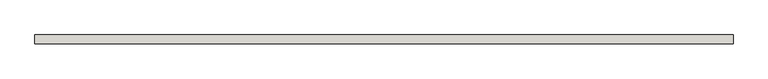
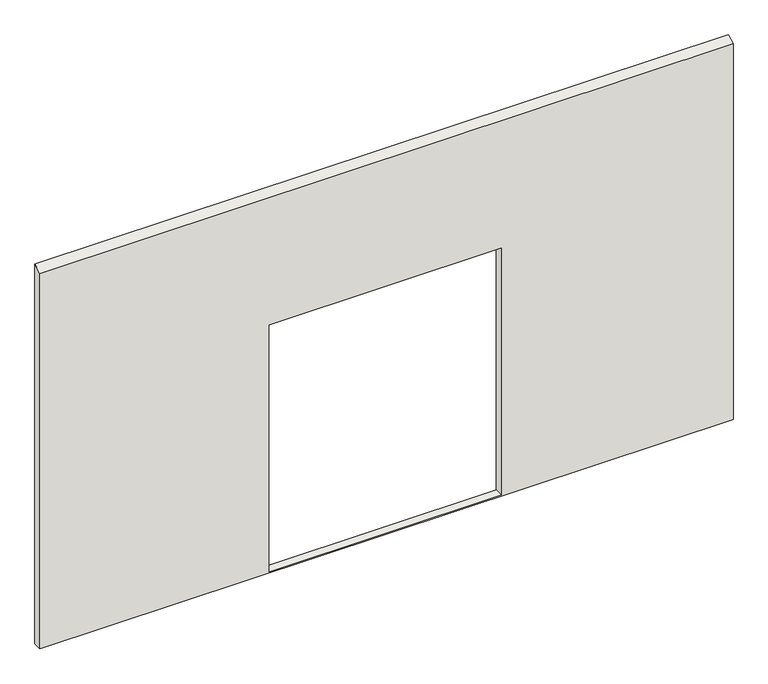
"""IFC4 building model written with IfcOpenShell, lengths in millimetres: wall geometry, 0_3d_modell."""

from ifc_helpers import new_model, si_unit, origin, place, context, project, spatial, faceted_brep, source, transform, mapped, element, save


def wall_7ed9d0b5(model_context):
    return source(origin(), model_context, "Body", "Brep", [
        faceted_brep([(1875.0, 70.0, 10.0), (1875.0, 70.0, 2145.0), (1875.0, 0.0, 2145.0), (1875.0, 0.0, 10.0), (3775.0, 70.0, 2145.0), (3775.0, 0.0, 2145.0), (3775.0, 70.0, 10.0), (3775.0, 0.0, 10.0), (5670.0, 0.0, 3247.913011), (5670.0, 70.0, 3283.5797924), (0.0, 70.0, 3283.5797924), (0.0, 0.0, 3247.913011), (0.0, 70.0, 0.0), (0.0, 0.0, 0.0), (5670.0, 0.0, 0.0), (5670.0, 70.0, 0.0)], [[[0, 1, 2, 3]], [[1, 4, 5, 2]], [[4, 6, 7, 5]], [[6, 0, 3, 7]], [[8, 9, 10, 11]], [[11, 10, 12, 13]], [[9, 8, 14, 15]], [[8, 11, 13, 14], [3, 2, 5, 7]], [[15, 12, 10, 9], [1, 0, 6, 4]], [[12, 15, 14, 13]]]),
    ])


if __name__ == "__main__":
    model = new_model("IFC4")
    model_context = context("Model", 3, world=origin())
    ifc_project = project(units=[si_unit("LENGTHUNIT", "METRE", prefix="MILLI")], contexts=[model_context])
    site = spatial("IfcSite", under=ifc_project)
    building = spatial("IfcBuilding", under=site)
    placement = place(None, origin())
    wall_shape = wall_7ed9d0b5(model_context)
    element("IfcWall", 1, ObjectType="0_3d_modell", at=placement, inside=building, context=model_context, shape_type="MappedRepresentation", body=[
        mapped(wall_shape, transform((0.0, 0.0, 0.0), x_axis=(1.0, 0.0, 0.0), y_axis=(0.0, 1.0, 0.0), z_axis=(0.0, 0.0, 1.0))),
    ])
    save(model, "model.ifc")

# Revit data of these elements
# Element 1 (IfcWall, "0_3d_modell")
#   Materials on its faces: "Glass_Simple"
# Materials
#   "Glass_Simple": class "Unassigned", colour RGB 255 255 255, transparency 0.9
